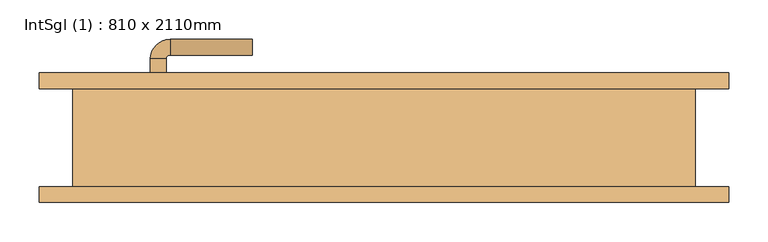
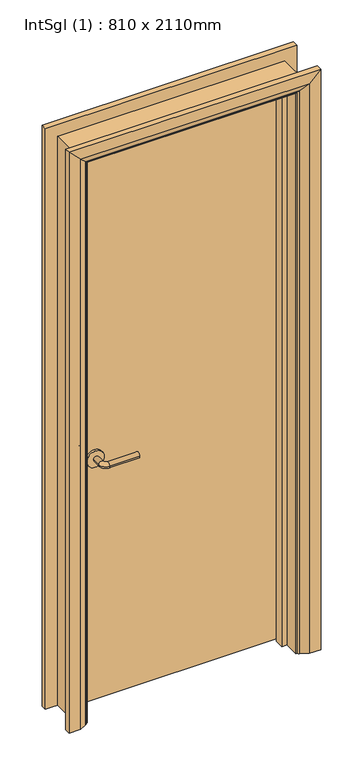
"""IFC4 building model written with IfcOpenShell, lengths in millimetres: door geometry, IntSgl (1) : 810 x 2110mm."""

from ifc_helpers import new_model, si_unit, point, frame, frame_2d, origin, place, context, project, spatial, polyline, circle_curve, ellipse_curve, trimmed, segment, composite_curve, outline, extrude, faceted_brep, source, transform, mapped, element, save
from ifc_brep_helpers import plane_surface, cylinder_surface, revolved_surface, advanced_brep


def intsgl_1_810_x_2110mm_60c2a13c(model_context):
    return source(origin(), model_context, "Body", "SolidModel", [
        advanced_brep(
        [(-298.0, 16.5, 900.0), (-278.0, 16.5, 900.0), (-278.0, -13.5, 900.0), (-298.0, -13.5, 900.0), (-273.0, -18.5, 900.0), (-273.0, -38.5, 900.0), (-168.0, -38.5, 900.0), (-168.0, -18.5, 900.0)],
        [
            (0, 1, circle_curve(frame((-288.0, 16.5, 900.0), z_axis=(0.0, 1.0, 0.0), x_axis=(1.0, 0.0, 0.0)), 10.0)),
            (1, 0, circle_curve(frame((-288.0, 16.5, 900.0), z_axis=(0.0, 1.0, 0.0), x_axis=(1.0, 0.0, 0.0)), 10.0)),
            (1, 2),
            (2, 3, circle_curve(frame((-288.0, -13.5, 900.0), z_axis=(0.0, 1.0, 0.0), x_axis=(1.0, 0.0, 0.0)), 10.0)),
            (3, 0),
            (3, 2, circle_curve(frame((-288.0, -13.5, 900.0), z_axis=(0.0, 1.0, 0.0), x_axis=(1.0, 0.0, 0.0)), 10.0)),
            (4, 5, circle_curve(frame((-273.0, -28.5, 900.0), z_axis=(-1.0, 0.0, 0.0), x_axis=(0.0, 1.0, 0.0)), 10.0)),
            (5, 3, circle_curve(frame((-273.0, -13.5, 900.0), z_axis=(0.0, 0.0, -1.0), x_axis=(-1.0, 0.0, 0.0)), 25.0)),
            (2, 4, circle_curve(frame((-273.0, -13.5, 900.0), z_axis=(0.0, 0.0, 1.0), x_axis=(-1.0, 0.0, 0.0)), 5.0)),
            (5, 4, circle_curve(frame((-273.0, -28.5, 900.0), z_axis=(-1.0, 0.0, 0.0), x_axis=(0.0, 1.0, 0.0)), 10.0)),
            (6, 7, circle_curve(frame((-168.0, -28.5, 900.0), z_axis=(1.0, 0.0, 0.0), x_axis=(0.0, 1.0, 0.0)), 10.0)),
            (7, 6, circle_curve(frame((-168.0, -28.5, 900.0), z_axis=(1.0, 0.0, 0.0), x_axis=(0.0, 1.0, 0.0)), 10.0)),
            (4, 7),
            (6, 5),
        ],
        [
            plane_surface(frame((-288.0, 16.5, 900.0), z_axis=(0.0, 1.0, 0.0), x_axis=(0.0, 0.0, 1.0))),
            cylinder_surface(frame((-288.0, 16.5, 900.0), z_axis=(0.0, 1.0, 0.0), x_axis=(1.0, 0.0, 0.0)), 10.0),
            revolved_surface(trimmed(ellipse_curve(frame((-288.0, -13.5, 900.0), z_axis=(0.0, -1.0, 0.0), x_axis=(1.0, 0.0, 0.0)), 10.0, 10.0), [point((-298.0, -13.5, 900.0))], [point((-278.0, -13.5, 900.0))], True, "CARTESIAN"), (-273.0, -13.5, 900.0), (0.0, 0.0, -1.0)),
            revolved_surface(trimmed(ellipse_curve(frame((-288.0, -13.5, 900.0), z_axis=(0.0, -1.0, 0.0), x_axis=(1.0, 0.0, 0.0)), 10.0, 10.0), [point((-278.0, -13.5, 900.0))], [point((-298.0, -13.5, 900.0))], True, "CARTESIAN"), (-273.0, -13.5, 900.0), (0.0, 0.0, -1.0)),
            plane_surface(frame((-168.0, -28.5, 900.0), z_axis=(1.0, 0.0, 0.0), x_axis=(0.0, 0.0, 1.0))),
            cylinder_surface(frame((-273.0, -28.5, 900.0), z_axis=(-1.0, 0.0, 0.0), x_axis=(0.0, 1.0, 0.0)), 10.0),
        ],
        [
            (0, [[1, 2]]),
            (1, [[3, 4, 5, -2]]),
            (1, [[-5, 6, -3, -1]]),
            (2, [[7, 8, -4, 9]]),
            (3, [[10, -9, -6, -8]]),
            (4, [[11, 12]]),
            (5, [[13, -11, 14, -7]]),
            (5, [[-14, -12, -13, -10]]),
        ],
    ),
        extrude(outline(composite_curve([segment(trimmed(circle_curve(frame_2d((900.0, -290.5)), 30.0), [point((900.0, -320.5))], [point((900.0, -260.5))], False, "CARTESIAN"), True, "CONTINUOUS"), segment(trimmed(circle_curve(frame_2d((900.0, -290.5)), 30.0), [point((900.0, -260.5))], [point((900.0, -320.5))], False, "CARTESIAN"), True, "CONTINUOUS")], self_intersect=False)), frame((0.0, 16.5, 0.0), z_axis=(0.0, 1.0, 0.0), x_axis=(0.0, 0.0, 1.0)), (0.0, 0.0, 1.0), 8.0),
        advanced_brep(
        [(-298.0, 70.5, 900.0), (-278.0, 70.5, 900.0), (-298.0, 100.5, 900.0), (-278.0, 100.5, 900.0), (-273.0, 105.5, 900.0), (-273.0, 125.5, 900.0), (-168.0, 125.5, 900.0), (-168.0, 105.5, 900.0)],
        [
            (0, 1, circle_curve(frame((-288.0, 70.5, 900.0), z_axis=(0.0, -1.0, 0.0), x_axis=(1.0, 0.0, 0.0)), 10.0)),
            (1, 0, circle_curve(frame((-288.0, 70.5, 900.0), z_axis=(0.0, -1.0, 0.0), x_axis=(1.0, 0.0, 0.0)), 10.0)),
            (0, 2),
            (2, 3, circle_curve(frame((-288.0, 100.5, 900.0), z_axis=(0.0, -1.0, 0.0), x_axis=(1.0, 0.0, 0.0)), 10.0)),
            (3, 1),
            (3, 2, circle_curve(frame((-288.0, 100.5, 900.0), z_axis=(0.0, -1.0, 0.0), x_axis=(1.0, 0.0, 0.0)), 10.0)),
            (4, 3, circle_curve(frame((-273.0, 100.5, 900.0), z_axis=(0.0, 0.0, 1.0), x_axis=(-1.0, 0.0, 0.0)), 5.0)),
            (2, 5, circle_curve(frame((-273.0, 100.5, 900.0), z_axis=(0.0, 0.0, -1.0), x_axis=(-1.0, 0.0, 0.0)), 25.0)),
            (5, 4, circle_curve(frame((-273.0, 115.5, 900.0), z_axis=(-1.0, 0.0, 0.0), x_axis=(0.0, -1.0, 0.0)), 10.0)),
            (4, 5, circle_curve(frame((-273.0, 115.5, 900.0), z_axis=(-1.0, 0.0, 0.0), x_axis=(0.0, -1.0, 0.0)), 10.0)),
            (6, 7, circle_curve(frame((-168.0, 115.5, 900.0), z_axis=(1.0, 0.0, 0.0), x_axis=(0.0, -1.0, 0.0)), 10.0)),
            (7, 6, circle_curve(frame((-168.0, 115.5, 900.0), z_axis=(1.0, 0.0, 0.0), x_axis=(0.0, -1.0, 0.0)), 10.0)),
            (5, 6),
            (7, 4),
        ],
        [
            plane_surface(frame((-288.0, 70.5, 900.0), z_axis=(0.0, -1.0, 0.0), x_axis=(0.0, 0.0, 1.0))),
            cylinder_surface(frame((-288.0, 70.5, 900.0), z_axis=(0.0, -1.0, 0.0), x_axis=(1.0, 0.0, 0.0)), 10.0),
            revolved_surface(trimmed(ellipse_curve(frame((-288.0, 100.5, 900.0), z_axis=(0.0, -1.0, 0.0), x_axis=(1.0, 0.0, 0.0)), 10.0, 10.0), [point((-298.0, 100.5, 900.0))], [point((-278.0, 100.5, 900.0))], True, "CARTESIAN"), (-273.0, 100.5, 900.0), (0.0, 0.0, -1.0)),
            revolved_surface(trimmed(ellipse_curve(frame((-288.0, 100.5, 900.0), z_axis=(0.0, -1.0, 0.0), x_axis=(1.0, 0.0, 0.0)), 10.0, 10.0), [point((-278.0, 100.5, 900.0))], [point((-298.0, 100.5, 900.0))], True, "CARTESIAN"), (-273.0, 100.5, 900.0), (0.0, 0.0, -1.0)),
            plane_surface(frame((-168.0, 115.5, 900.0), z_axis=(1.0, 0.0, 0.0), x_axis=(0.0, 0.0, 1.0))),
            cylinder_surface(frame((-273.0, 115.5, 900.0), z_axis=(-1.0, 0.0, 0.0), x_axis=(0.0, -1.0, 0.0)), 10.0),
        ],
        [
            (0, [[1, 2]]),
            (1, [[-1, 3, 4, 5]]),
            (1, [[-2, -5, 6, -3]]),
            (2, [[7, -4, 8, 9]]),
            (3, [[-8, -6, -7, 10]]),
            (4, [[11, 12]]),
            (5, [[-9, 13, -12, 14]]),
            (5, [[-10, -14, -11, -13]]),
        ],
    ),
        extrude(outline(composite_curve([segment(trimmed(circle_curve(frame_2d((900.0, -290.5)), 30.0), [point((900.0, -320.5))], [point((900.0, -260.5))], False, "CARTESIAN"), True, "CONTINUOUS"), segment(trimmed(circle_curve(frame_2d((900.0, -290.5)), 30.0), [point((900.0, -260.5))], [point((900.0, -320.5))], False, "CARTESIAN"), True, "CONTINUOUS")], self_intersect=False)), frame((0.0, 62.5, 0.0), z_axis=(0.0, 1.0, 0.0), x_axis=(0.0, 0.0, 1.0)), (0.0, 0.0, 1.0), 8.0),
        extrude(outline(polyline([(363.0, 24.5), (-363.0, 24.5), (-363.0, 62.5), (363.0, 62.5), (363.0, 24.5)])), frame((0.0, 0.0, 8.0), z_axis=(0.0, 0.0, 1.0), x_axis=(1.0, 0.0, 0.0)), (0.0, 0.0, 1.0), 2060.0),
        advanced_brep(
        [(440.0, 82.5, 0.0), (440.0, 62.5, 0.0), (370.0, 62.5, 0.0), (374.0, 68.5, 0.0), (400.0, 82.5, 0.0), (440.0, 82.5, 2145.0), (440.0, 62.5, 2145.0), (-440.0, 62.5, 2145.0), (-440.0, 62.5, 0.0), (-370.0, 62.5, 0.0), (-370.0, 62.5, 2075.0), (370.0, 62.5, 2075.0), (374.0, 68.5, 2079.0), (400.0, 82.5, 2105.0), (-400.0, 82.5, 2105.0), (-400.0, 82.5, 0.0), (-440.0, 82.5, 0.0), (-440.0, 82.5, 2145.0), (-374.0, 68.5, 2079.0), (-374.0, 68.5, 0.0)],
        [
            (0, 1),
            (1, 2),
            (2, 3, circle_curve(frame((378.0, 61.5, 0.0), z_axis=(0.0, 0.0, -1.0), x_axis=(1.0, 0.0, 0.0)), 8.0622577)),
            (3, 4),
            (4, 0),
            (0, 5),
            (5, 6),
            (6, 1),
            (6, 7),
            (7, 8),
            (8, 9),
            (9, 10),
            (10, 11),
            (11, 2),
            (11, 12, ellipse_curve(frame((378.0, 61.5, 2083.0), z_axis=(0.7071067811865475, 0.0, -0.7071067811865475), x_axis=(-0.7071067811865474, 0.0, -0.7071067811865476)), 11.4017543, 8.0622577)),
            (12, 3),
            (12, 13),
            (13, 4),
            (13, 14),
            (14, 15),
            (15, 16),
            (16, 17),
            (17, 5),
            (17, 7),
            (10, 18, ellipse_curve(frame((-378.0, 61.5, 2083.0), z_axis=(0.7071067811865475, 0.0, 0.7071067811865475), x_axis=(0.7071067811865476, 0.0, -0.7071067811865474)), 11.4017543, 8.0622577)),
            (18, 12),
            (18, 14),
            (15, 19),
            (19, 9, circle_curve(frame((-378.0, 61.5, 0.0), z_axis=(0.0, 0.0, -1.0), x_axis=(-1.0, 0.0, 0.0)), 8.0622577)),
            (8, 16),
            (19, 18),
        ],
        [
            plane_surface(frame((370.0, 62.5, 0.0), z_axis=(0.0, 0.0, -1.0), x_axis=(0.0, -1.0, 0.0))),
            plane_surface(frame((440.0, 82.5, 0.0), z_axis=(1.0, 0.0, 0.0), x_axis=(0.0, 0.0, 1.0))),
            plane_surface(frame((440.0, 62.5, 0.0), z_axis=(0.0, -1.0, 0.0), x_axis=(0.0, 0.0, 1.0))),
            cylinder_surface(frame((378.0, 61.5, 0.0), z_axis=(0.0, 0.0, -1.0), x_axis=(1.0, 0.0, 0.0)), 8.0622577),
            plane_surface(frame((374.0, 68.5, 0.0), z_axis=(-0.4740998230350126, 0.880471099922178, 0.0), x_axis=(0.0, 0.0, 1.0))),
            plane_surface(frame((400.0, 82.5, 0.0), z_axis=(0.0, 1.0, 0.0), x_axis=(0.0, 0.0, 1.0))),
            plane_surface(frame((440.0, 82.5, 2145.0), z_axis=(0.0, 0.0, 1.0), x_axis=(-1.0, 0.0, 0.0))),
            cylinder_surface(frame((370.0, 61.5, 2083.0), z_axis=(1.0, 0.0, 0.0), x_axis=(0.0, 0.0, 1.0)), 8.0622577),
            plane_surface(frame((374.0, 68.5, 2079.0), z_axis=(0.0, 0.8804710999221764, -0.4740998230350154), x_axis=(-1.0, 0.0, 0.0))),
            plane_surface(frame((-370.0, 62.5, 0.0), z_axis=(0.0, 0.0, -1.0), x_axis=(0.0, -1.0, 0.0))),
            plane_surface(frame((-440.0, 82.5, 2145.0), z_axis=(-1.0, 0.0, 0.0), x_axis=(0.0, 0.0, -1.0))),
            cylinder_surface(frame((-378.0, 61.5, 2075.0), z_axis=(0.0, 0.0, 1.0), x_axis=(-1.0, 0.0, 0.0)), 8.0622577),
            plane_surface(frame((-374.0, 68.5, 2079.0), z_axis=(0.47409982303501824, 0.8804710999221749, 0.0), x_axis=(0.0, 0.0, -1.0))),
        ],
        [
            (0, [[1, 2, 3, 4, 5]]),
            (1, [[-1, 6, 7, 8]]),
            (2, [[-2, -8, 9, 10, 11, 12, 13, 14]]),
            (3, [[-3, -14, 15, 16]]),
            (4, [[-4, -16, 17, 18]]),
            (5, [[-5, -18, 19, 20, 21, 22, 23, -6]]),
            (6, [[-7, -23, 24, -9]]),
            (7, [[-15, -13, 25, 26]]),
            (8, [[-17, -26, 27, -19]]),
            (9, [[-21, 28, 29, -11, 30]]),
            (10, [[-24, -22, -30, -10]]),
            (11, [[-25, -12, -29, 31]]),
            (12, [[-27, -31, -28, -20]]),
        ],
    ),
        extrude(outline(polyline([(0.0, -365.0), (0.0, -346.0), (2051.0, -346.0), (2051.0, 346.0), (0.0, 346.0), (0.0, 365.0), (2070.0, 365.0), (2070.0, -365.0), (0.0, -365.0)])), frame((0.0, -9.5, 0.0), z_axis=(0.0, 1.0, 0.0), x_axis=(0.0, 0.0, 1.0)), (0.0, 0.0, 1.0), 32.0),
        advanced_brep(
        [(-440.0, -82.5, 0.0), (-440.0, -62.5, 0.0), (-370.0, -62.5, 0.0), (-374.0, -68.5, 0.0), (-400.0, -82.5, 0.0), (-440.0, -82.5, 2145.0), (-440.0, -62.5, 2145.0), (-370.0, -62.5, 2075.0), (-374.0, -68.5, 2079.0), (-400.0, -82.5, 2105.0), (440.0, -82.5, 2145.0), (440.0, -62.5, 2145.0), (370.0, -62.5, 2075.0), (374.0, -68.5, 2079.0), (400.0, -82.5, 2105.0), (440.0, -82.5, 0.0), (400.0, -82.5, 0.0), (374.0, -68.5, 0.0), (370.0, -62.5, 0.0), (440.0, -62.5, 0.0)],
        [
            (0, 1),
            (1, 2),
            (2, 3, circle_curve(frame((-378.0, -61.5, 0.0), z_axis=(0.0, 0.0, -1.0), x_axis=(-1.0, 0.0, 0.0)), 8.0622577)),
            (3, 4),
            (4, 0),
            (0, 5),
            (5, 6),
            (6, 1),
            (6, 7),
            (7, 2),
            (7, 8, ellipse_curve(frame((-378.0, -61.5, 2083.0), z_axis=(-0.7071067811865475, 0.0, -0.7071067811865475), x_axis=(0.7071067811865474, 0.0, -0.7071067811865476)), 11.4017543, 8.0622577)),
            (8, 3),
            (8, 9),
            (9, 4),
            (9, 5),
            (5, 10),
            (10, 11),
            (11, 6),
            (11, 12),
            (12, 7),
            (12, 13, ellipse_curve(frame((378.0, -61.5, 2083.0), z_axis=(-0.7071067811865475, 0.0, 0.7071067811865475), x_axis=(-0.7071067811865476, 0.0, -0.7071067811865474)), 11.4017543, 8.0622577)),
            (13, 8),
            (13, 14),
            (14, 9),
            (14, 10),
            (15, 16),
            (16, 17),
            (17, 18, circle_curve(frame((378.0, -61.5, 0.0), z_axis=(0.0, 0.0, -1.0), x_axis=(1.0, 0.0, 0.0)), 8.0622577)),
            (18, 19),
            (19, 15),
            (10, 15),
            (19, 11),
            (18, 12),
            (17, 13),
            (16, 14),
        ],
        [
            plane_surface(frame((-370.0, -135.3010989, 0.0), z_axis=(0.0, 0.0, -1.0), x_axis=(1.0, 0.0, 0.0))),
            plane_surface(frame((-440.0, -82.5, 0.0), z_axis=(-1.0, 0.0, 0.0), x_axis=(0.0, 0.0, 1.0))),
            plane_surface(frame((-440.0, -62.5, 0.0), z_axis=(0.0, 1.0, 0.0), x_axis=(0.0, 0.0, 1.0))),
            cylinder_surface(frame((-378.0, -61.5, 0.0), z_axis=(0.0, 0.0, -1.0), x_axis=(-1.0, 0.0, 0.0)), 8.0622577),
            plane_surface(frame((-374.0, -68.5, 0.0), z_axis=(0.4740998230350183, -0.8804710999221749, 0.0), x_axis=(0.0, 0.0, 1.0))),
            plane_surface(frame((-400.0, -82.5, 0.0), z_axis=(0.0, -1.0, 0.0), x_axis=(0.0, 0.0, 1.0))),
            plane_surface(frame((-440.0, -82.5, 2145.0), z_axis=(0.0, 0.0, 1.0), x_axis=(1.0, 0.0, 0.0))),
            plane_surface(frame((-440.0, -62.5, 2145.0), z_axis=(0.0, 1.0, 0.0), x_axis=(1.0, 0.0, 0.0))),
            cylinder_surface(frame((-370.0, -61.5, 2083.0), z_axis=(-1.0, 0.0, 0.0), x_axis=(0.0, 0.0, 1.0)), 8.0622577),
            plane_surface(frame((-374.0, -68.5, 2079.0), z_axis=(0.0, -0.8804710999221749, -0.4740998230350183), x_axis=(1.0, 0.0, 0.0))),
            plane_surface(frame((-400.0, -82.5, 2105.0), z_axis=(0.0, -1.0, 0.0), x_axis=(1.0, 0.0, 0.0))),
            plane_surface(frame((370.0, -135.3010989, 0.0), z_axis=(0.0, 0.0, -1.0), x_axis=(-1.0, 0.0, 0.0))),
            plane_surface(frame((440.0, -82.5, 2145.0), z_axis=(1.0, 0.0, 0.0), x_axis=(0.0, 0.0, -1.0))),
            plane_surface(frame((440.0, -62.5, 2145.0), z_axis=(0.0, 1.0, 0.0), x_axis=(0.0, 0.0, -1.0))),
            cylinder_surface(frame((378.0, -61.5, 2075.0), z_axis=(0.0, 0.0, 1.0), x_axis=(1.0, 0.0, 0.0)), 8.0622577),
            plane_surface(frame((374.0, -68.5, 2079.0), z_axis=(-0.4740998230350183, -0.8804710999221749, 0.0), x_axis=(0.0, 0.0, -1.0))),
            plane_surface(frame((400.0, -82.5, 2105.0), z_axis=(0.0, -1.0, 0.0), x_axis=(0.0, 0.0, -1.0))),
        ],
        [
            (0, [[1, 2, 3, 4, 5]]),
            (1, [[-1, 6, 7, 8]]),
            (2, [[-2, -8, 9, 10]]),
            (3, [[-3, -10, 11, 12]]),
            (4, [[-4, -12, 13, 14]]),
            (5, [[-5, -14, 15, -6]]),
            (6, [[-7, 16, 17, 18]]),
            (7, [[-9, -18, 19, 20]]),
            (8, [[-11, -20, 21, 22]]),
            (9, [[-13, -22, 23, 24]]),
            (10, [[-15, -24, 25, -16]]),
            (11, [[26, 27, 28, 29, 30]]),
            (12, [[-17, 31, -30, 32]]),
            (13, [[-19, -32, -29, 33]]),
            (14, [[-21, -33, -28, 34]]),
            (15, [[-23, -34, -27, 35]]),
            (16, [[-25, -35, -26, -31]]),
        ],
    ),
        faceted_brep([(-365.0, 62.5, 0.0), (-365.0, -62.5, 0.0), (-397.0, -62.5, 0.0), (-397.0, 62.5, 0.0), (-365.0, 62.5, 2070.0), (-365.0, -62.5, 2070.0), (-397.0, -62.5, 2102.0), (-397.0, 62.5, 2102.0), (365.0, 62.5, 2070.0), (365.0, -62.5, 2070.0), (397.0, -62.5, 2102.0), (397.0, 62.5, 2102.0), (365.0, 62.5, 0.0), (397.0, 62.5, 0.0), (397.0, -62.5, 0.0), (365.0, -62.5, 0.0)], [[[0, 1, 2, 3]], [[1, 0, 4, 5]], [[2, 1, 5, 6]], [[3, 2, 6, 7]], [[0, 3, 7, 4]], [[5, 4, 8, 9]], [[6, 5, 9, 10]], [[7, 6, 10, 11]], [[4, 7, 11, 8]], [[12, 13, 14, 15]], [[9, 8, 12, 15]], [[10, 9, 15, 14]], [[11, 10, 14, 13]], [[8, 11, 13, 12]]]),
    ])


if __name__ == "__main__":
    model = new_model("IFC4")
    model_context = context("Model", 3, world=origin())
    ifc_project = project(units=[si_unit("LENGTHUNIT", "METRE", prefix="MILLI")], contexts=[model_context])
    site = spatial("IfcSite", under=ifc_project)
    building = spatial("IfcBuilding", under=site)
    placement = place(None, origin())
    intsgl_1_810_x_2110mm_shape = intsgl_1_810_x_2110mm_60c2a13c(model_context)
    element("IfcDoor", 1, ObjectType="IntSgl (1) : 810 x 2110mm", at=placement, inside=building, context=model_context, shape_type="MappedRepresentation", body=[
        mapped(intsgl_1_810_x_2110mm_shape, transform((0.0, 0.0, 0.0), x_axis=(1.0, 0.0, 0.0), y_axis=(0.0, 1.0, 0.0), z_axis=(0.0, 0.0, 1.0))),
    ])
    save(model, "model.ifc")

# Revit data of these elements
# Type "IntSgl (1) : 810 x 2110mm"
#   Construction Type Id = "MDOOR"
#   Analytic Construction = "Metal"
#   Type Mark = "42"
#   Type Comments = "Internal Single"
#   Operation = "SingleSwingRight"
#   Manufacturer = "Revit"
#   Keynote = "L20"
#   Description = "Internal Single Door"
#   Visual Light Transmittance = 0
#   Solar Heat Gain Coefficient = 0
#   Heat Transfer Coefficient (U) = 3.7021 W/(m²·K)
#   UnderCut = 8 mm
#   Tolerance = 2 mm
#   Thickness = 38 mm
#   Structural Tolerance = 8 mm
#   StopDepth = 32 mm
#   Stop Thickness = 19 mm
#   Rough Width = 810 mm
#   Rough Height = 2110 mm
#   Height to Top Lock Rail = 1000 mm
#   Handle Z Distance = 900 mm
#   Handle X Distance = 75 mm
#   Frame Thickness = 32 mm
#   Door Panel Width = 726 mm
#   Door Panel Thickness = 38 mm
#   Door Panel Offset = 0 mm
#   Height = 2110 mm
#   Width = 810 mm
#   Door Panel Height = 2060 mm
#   Architrave Setback = 5 mm
#   Function = 0
#   Vis - Ironmongery = yes
#   Material Ironmongery = Door - Handle
#   Material Frame = Door - Frame/Mullion (1)
#   Material Door = Door - Panel
#   Material Architrave = Door - Architrave
#   Wall Closure = (empty or 0)
# Element 1 (IfcDoor, "IntSgl (1) : 810 x 2110mm")
#   Materials on its faces: "Door - Architrave", "Door - Handle", "Door - Frame/Mullion (1)", "Door - Panel"
# Materials
#   "Door - Handle": class "Miscellaneous", colour RGB 0 0 0, transparency 0, Keynote = "P21"
#   "Door - Frame/Mullion (1)": class "Wood", colour RGB 212 179 113, transparency 0, Keynote = "L20", Cost = 0
#   "Door - Panel": class "Wood", colour RGB 210 159 95, transparency 0, Keynote = "L20"
#   "Door - Architrave": class "Wood", colour RGB 154 90 5, transparency 0, Keynote = "P20"
